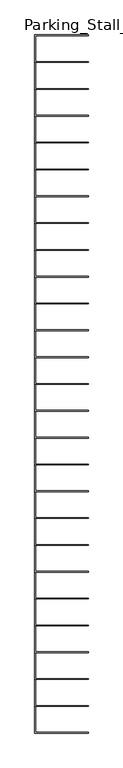
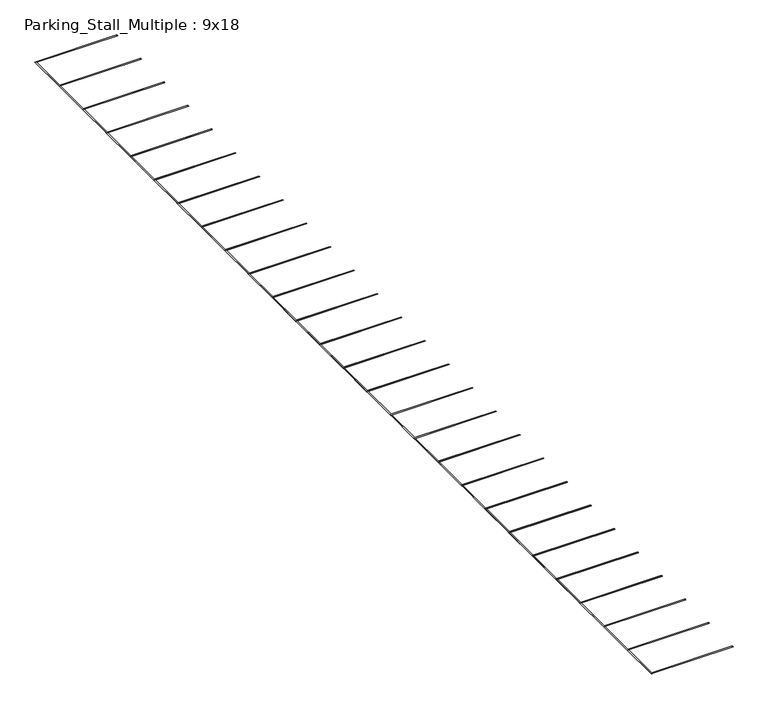
"""IFC4 building model written with IfcOpenShell, lengths in millimetres: proxy geometry, Parking_Stall_Multiple : 9x18."""

import ifcopenshell
import ifcopenshell.guid

model = None  # the IFC model being written
_history = None  # IfcOwnerHistory: only IFC2X3 demands one
_inside = {}  # id of a spatial element -> (the spatial element, [elements in it])
_under = {}  # id of a project, library or spatial element -> (it, [spatial elements below it])
_declared = {}  # id of a project -> (the project, [libraries it declares])
_typed = {}  # id of a type object -> (the type object, [elements of that type])
_made_of = {}  # id of a material, layer set ... -> (it, [elements and type objects made of it])


def new_model(schema):
    """Start an empty IFC model of exactly this schema.

    Asked for "IFC4X3", IfcOpenShell would pick the latest addendum, in which some entities
    have other attributes; the version numbers below select the first issue.
    IFC2X3 requires an IfcOwnerHistory on every rooted entity: one is made here for all.
    """
    global model, _history
    if schema == "IFC4X3":
        model = ifcopenshell.file(schema_version=(4, 3, 0, 0))
    else:
        model = ifcopenshell.file(schema=schema)
    _inside.clear()
    _under.clear()
    _declared.clear()
    _typed.clear()
    _made_of.clear()
    _history = None
    if model.schema == "IFC2X3":
        org = make("IfcOrganization", Name="unknown")
        user = make(
            "IfcPersonAndOrganization",
            ThePerson=make("IfcPerson", FamilyName="unknown"),
            TheOrganization=org,
        )
        app = make(
            "IfcApplication",
            ApplicationDeveloper=org,
            Version="unknown",
            ApplicationFullName="unknown",
            ApplicationIdentifier="unknown",
        )
        _history = make(
            "IfcOwnerHistory",
            OwningUser=user,
            OwningApplication=app,
            ChangeAction="ADDED",
            CreationDate=0,
        )
    return model


def make(cls, **values):
    """One entity of the class cls with the attributes given. An attribute that is None is left unset."""
    return model.create_entity(
        cls, **{name: value for name, value in values.items() if value is not None}
    )


def rooted(cls, **values):
    """An entity with a GlobalId (a new one), such as an element, a storey or a relation."""
    return make(cls, GlobalId=ifcopenshell.guid.new(), OwnerHistory=_history, **values)


def si_unit(unit_type, name, prefix=None):
    """IfcSIUnit, for example si_unit("LENGTHUNIT", "METRE", prefix="MILLI")."""
    return make("IfcSIUnit", UnitType=unit_type, Prefix=prefix, Name=name)


def assignment(units):
    """IfcUnitAssignment: the units of a project."""
    return None if units is None else make("IfcUnitAssignment", Units=units)


def point(xyz):
    """IfcCartesianPoint."""
    return None if xyz is None else make("IfcCartesianPoint", Coordinates=xyz)


def direction(xyz):
    """IfcDirection."""
    return None if xyz is None else make("IfcDirection", DirectionRatios=xyz)


def frame(location, z_axis=None, x_axis=None):
    """IfcAxis2Placement3D, a coordinate frame: its origin and axes. An axis left out is left unset."""
    return make(
        "IfcAxis2Placement3D",
        Location=point(location),
        Axis=direction(z_axis),
        RefDirection=direction(x_axis),
    )


def origin():
    """The frame at (0, 0, 0) with its axes left unset."""
    return frame((0.0, 0.0, 0.0))


def origin_with_axes():
    """The frame at (0, 0, 0) with the z axis (0, 0, 1) and the x axis (1, 0, 0) written out."""
    return frame((0.0, 0.0, 0.0), z_axis=(0.0, 0.0, 1.0), x_axis=(1.0, 0.0, 0.0))


def place(relative_to, where):
    """IfcLocalPlacement: puts the frame where relative to a parent placement (None: the world)."""
    return make(
        "IfcLocalPlacement", PlacementRelTo=relative_to, RelativePlacement=where
    )


def context(
    kind, dimensions, precision=None, world=None, true_north=None, identifier=None
):
    """IfcGeometricRepresentationContext, for example the 3D "Model" context."""
    return make(
        "IfcGeometricRepresentationContext",
        ContextIdentifier=identifier,
        ContextType=kind,
        CoordinateSpaceDimension=dimensions,
        Precision=precision,
        WorldCoordinateSystem=world,
        TrueNorth=true_north,
    )


def project(units=None, contexts=None):
    """IfcProject with its units and contexts."""
    return rooted(
        "IfcProject",
        Name="project",
        RepresentationContexts=contexts,
        UnitsInContext=assignment(units),
    )


def spatial(cls, under=None, at=None, **own):
    """A site, building, storey or space (cls), placed at a placement, below another one or the project."""
    s = rooted(cls, ObjectPlacement=at, **own)
    if under is not None:
        _under.setdefault(under.id(), (under, []))[1].append(s)
    return s


def polyline(points):
    """IfcPolyline through the points."""
    return make("IfcPolyline", Points=[point(p) for p in points])


def outline(outer, holes=None, kind="AREA"):
    """IfcArbitraryClosedProfileDef: a profile drawn as a closed curve; with holes, ...WithVoids."""
    if holes is None:
        return make("IfcArbitraryClosedProfileDef", ProfileType=kind, OuterCurve=outer)
    return make(
        "IfcArbitraryProfileDefWithVoids",
        ProfileType=kind,
        OuterCurve=outer,
        InnerCurves=holes,
    )


def extrude(swept, where, along, depth):
    """IfcExtrudedAreaSolid: the profile swept, set in the frame where, extruded along a direction by depth."""
    return make(
        "IfcExtrudedAreaSolid",
        SweptArea=swept,
        Position=where,
        ExtrudedDirection=direction(along),
        Depth=depth,
    )


def shape(context_of_items, identifier, shape_type, items):
    """IfcShapeRepresentation: the items that make up one representation, for example the "Body"."""
    return make(
        "IfcShapeRepresentation",
        ContextOfItems=context_of_items,
        RepresentationIdentifier=identifier,
        RepresentationType=shape_type,
        Items=items,
    )


def source(mapping_origin, context_of_items, identifier, shape_type, items):
    """IfcRepresentationMap: a shape defined once, which mapped items show again and again."""
    return make(
        "IfcRepresentationMap",
        MappingOrigin=mapping_origin,
        MappedRepresentation=shape(context_of_items, identifier, shape_type, items),
    )


def transform(
    local_origin,
    x_axis=None,
    y_axis=None,
    z_axis=None,
    scale=None,
    scale2=None,
    scale3=None,
    uniform=True,
):
    """IfcCartesianTransformationOperator3D, or its non-uniform kind. x_axis, y_axis, z_axis: its Axis1, 2, 3."""
    if uniform:
        return make(
            "IfcCartesianTransformationOperator3D",
            Axis1=direction(x_axis),
            Axis2=direction(y_axis),
            LocalOrigin=point(local_origin),
            Scale=scale,
            Axis3=direction(z_axis),
        )
    return make(
        "IfcCartesianTransformationOperator3DnonUniform",
        Axis1=direction(x_axis),
        Axis2=direction(y_axis),
        LocalOrigin=point(local_origin),
        Scale=scale,
        Axis3=direction(z_axis),
        Scale2=scale2,
        Scale3=scale3,
    )


def mapped(mapping_source, mapping_target):
    """IfcMappedItem: shows the shape of a source again, moved by a transform."""
    return make(
        "IfcMappedItem", MappingSource=mapping_source, MappingTarget=mapping_target
    )


def made_of(thing, what):
    """Note that an element or type object is made of a material, layer set ...; save() writes the relation."""
    if what is not None:
        _made_of.setdefault(what.id(), (what, []))[1].append(thing)
    return thing


def element(
    cls,
    number,
    at=None,
    inside=None,
    cuts=None,
    type_object=None,
    material=None,
    context=None,
    identifier="Body",
    shape_type=None,
    held_by="IfcProductDefinitionShape",
    body=None,
    shapes=None,
    **own,
):
    """One element of the class cls, such as IfcWall. Its Tag is "e" and its number.

    at: its placement. inside: the storey or other place that contains it. cuts: it is an
    opening in that element (IfcRelVoidsElement). A single representation is given by context,
    identifier, shape_type and body (its items); several are given by shapes. held_by: the class
    of the entity that holds the representations. save() writes the other relations.
    """
    e = rooted(cls, Tag="e%d" % number, ObjectPlacement=at, **own)
    if body is not None:
        shapes = [shape(context, identifier, shape_type, body)]
    if shapes is not None:
        e.Representation = make(held_by, Representations=shapes)
    if inside is not None:
        _inside.setdefault(inside.id(), (inside, []))[1].append(e)
    if cuts is not None:
        rooted(
            "IfcRelVoidsElement", RelatingBuildingElement=cuts, RelatedOpeningElement=e
        )
    if type_object is not None:
        _typed.setdefault(type_object.id(), (type_object, []))[1].append(e)
    return made_of(e, material)


def aggregate(whole, parts):
    """IfcRelAggregates: a whole, such as a stair, and the parts it consists of."""
    return rooted("IfcRelAggregates", RelatingObject=whole, RelatedObjects=parts)


def save(model, path):
    """Write the relations noted so far, then the file.

    IfcRelAggregates (storeys below a building ...), IfcRelContainedInSpatialStructure (elements
    in a storey), IfcRelDefinesByType, IfcRelAssociatesMaterial and IfcRelDeclares: one each for
    every whole, place, type object, material and project.
    """
    for whole, parts in _under.values():
        aggregate(whole, parts)
    for where, things in _inside.values():
        rooted(
            "IfcRelContainedInSpatialStructure",
            RelatedElements=things,
            RelatingStructure=where,
        )
    for kind, things in _typed.values():
        rooted("IfcRelDefinesByType", RelatedObjects=things, RelatingType=kind)
    for what, things in _made_of.values():
        rooted("IfcRelAssociatesMaterial", RelatedObjects=things, RelatingMaterial=what)
    for by, libraries in _declared.values():
        rooted("IfcRelDeclares", RelatingContext=by, RelatedDefinitions=libraries)
    model.write(path)


def parking_stall_multiple_9x18_b666618d(model_context):
    return source(origin(), model_context, "Body", "SweptSolid", [
        extrude(outline(polyline([(5486.4, 68580.0), (0.0, 68580.0), (0.0, 71399.4), (5486.4, 71399.4), (5486.4, 71323.2), (76.2, 71323.2), (76.2, 68656.2), (5486.4, 68656.2), (5486.4, 68580.0)])), origin_with_axes(), (0.0, 0.0, 1.0), 6.35),
        extrude(outline(polyline([(5486.4, 65836.8), (0.0, 65836.8), (0.0, 68656.2), (5486.4, 68656.2), (5486.4, 68580.0), (76.2, 68580.0), (76.2, 65913.0), (5486.4, 65913.0), (5486.4, 65836.8)])), origin_with_axes(), (0.0, 0.0, 1.0), 6.35),
        extrude(outline(polyline([(5486.4, 63093.6), (0.0, 63093.6), (0.0, 65913.0), (5486.4, 65913.0), (5486.4, 65836.8), (76.2, 65836.8), (76.2, 63169.8), (5486.4, 63169.8), (5486.4, 63093.6)])), origin_with_axes(), (0.0, 0.0, 1.0), 6.35),
        extrude(outline(polyline([(5486.4, 60350.4), (0.0, 60350.4), (0.0, 63169.8), (5486.4, 63169.8), (5486.4, 63093.6), (76.2, 63093.6), (76.2, 60426.6), (5486.4, 60426.6), (5486.4, 60350.4)])), origin_with_axes(), (0.0, 0.0, 1.0), 6.35),
        extrude(outline(polyline([(5486.4, 57607.2), (0.0, 57607.2), (0.0, 60426.6), (5486.4, 60426.6), (5486.4, 60350.4), (76.2, 60350.4), (76.2, 57683.4), (5486.4, 57683.4), (5486.4, 57607.2)])), origin_with_axes(), (0.0, 0.0, 1.0), 6.35),
        extrude(outline(polyline([(5486.4, 54864.0), (0.0, 54864.0), (0.0, 57683.4), (5486.4, 57683.4), (5486.4, 57607.2), (76.2, 57607.2), (76.2, 54940.2), (5486.4, 54940.2), (5486.4, 54864.0)])), origin_with_axes(), (0.0, 0.0, 1.0), 6.35),
        extrude(outline(polyline([(5486.4, 52120.8), (0.0, 52120.8), (0.0, 54940.2), (5486.4, 54940.2), (5486.4, 54864.0), (76.2, 54864.0), (76.2, 52197.0), (5486.4, 52197.0), (5486.4, 52120.8)])), origin_with_axes(), (0.0, 0.0, 1.0), 6.35),
        extrude(outline(polyline([(5486.4, 49377.6), (0.0, 49377.6), (0.0, 52197.0), (5486.4, 52197.0), (5486.4, 52120.8), (76.2, 52120.8), (76.2, 49453.8), (5486.4, 49453.8), (5486.4, 49377.6)])), origin_with_axes(), (0.0, 0.0, 1.0), 6.35),
        extrude(outline(polyline([(5486.4, 46634.4), (0.0, 46634.4), (0.0, 49453.8), (5486.4, 49453.8), (5486.4, 49377.6), (76.2, 49377.6), (76.2, 46710.6), (5486.4, 46710.6), (5486.4, 46634.4)])), origin_with_axes(), (0.0, 0.0, 1.0), 6.35),
        extrude(outline(polyline([(5486.4, 43891.2), (0.0, 43891.2), (0.0, 46710.6), (5486.4, 46710.6), (5486.4, 46634.4), (76.2, 46634.4), (76.2, 43967.4), (5486.4, 43967.4), (5486.4, 43891.2)])), origin_with_axes(), (0.0, 0.0, 1.0), 6.35),
        extrude(outline(polyline([(5486.4, 41148.0), (0.0, 41148.0), (0.0, 43967.4), (5486.4, 43967.4), (5486.4, 43891.2), (76.2, 43891.2), (76.2, 41224.2), (5486.4, 41224.2), (5486.4, 41148.0)])), origin_with_axes(), (0.0, 0.0, 1.0), 6.35),
        extrude(outline(polyline([(5486.4, 38404.8), (0.0, 38404.8), (0.0, 41224.2), (5486.4, 41224.2), (5486.4, 41148.0), (76.2, 41148.0), (76.2, 38481.0), (5486.4, 38481.0), (5486.4, 38404.8)])), origin_with_axes(), (0.0, 0.0, 1.0), 6.35),
        extrude(outline(polyline([(5486.4, 35661.6), (0.0, 35661.6), (0.0, 38481.0), (5486.4, 38481.0), (5486.4, 38404.8), (76.2, 38404.8), (76.2, 35737.8), (5486.4, 35737.8), (5486.4, 35661.6)])), origin_with_axes(), (0.0, 0.0, 1.0), 6.35),
        extrude(outline(polyline([(5486.4, 32918.4), (0.0, 32918.4), (0.0, 35737.8), (5486.4, 35737.8), (5486.4, 35661.6), (76.2, 35661.6), (76.2, 32994.6), (5486.4, 32994.6), (5486.4, 32918.4)])), origin_with_axes(), (0.0, 0.0, 1.0), 6.35),
        extrude(outline(polyline([(5486.4, 30175.2), (0.0, 30175.2), (0.0, 32994.6), (5486.4, 32994.6), (5486.4, 32918.4), (76.2, 32918.4), (76.2, 30251.4), (5486.4, 30251.4), (5486.4, 30175.2)])), origin_with_axes(), (0.0, 0.0, 1.0), 6.35),
        extrude(outline(polyline([(5486.4, 27432.0), (0.0, 27432.0), (0.0, 30251.4), (5486.4, 30251.4), (5486.4, 30175.2), (76.2, 30175.2), (76.2, 27508.2), (5486.4, 27508.2), (5486.4, 27432.0)])), origin_with_axes(), (0.0, 0.0, 1.0), 6.35),
        extrude(outline(polyline([(5486.4, 24688.8), (0.0, 24688.8), (0.0, 27508.2), (5486.4, 27508.2), (5486.4, 27432.0), (76.2, 27432.0), (76.2, 24765.0), (5486.4, 24765.0), (5486.4, 24688.8)])), origin_with_axes(), (0.0, 0.0, 1.0), 6.35),
        extrude(outline(polyline([(5486.4, 21945.6), (0.0, 21945.6), (0.0, 24765.0), (5486.4, 24765.0), (5486.4, 24688.8), (76.2, 24688.8), (76.2, 22021.8), (5486.4, 22021.8), (5486.4, 21945.6)])), origin_with_axes(), (0.0, 0.0, 1.0), 6.35),
        extrude(outline(polyline([(5486.4, 19202.4), (0.0, 19202.4), (0.0, 22021.8), (5486.4, 22021.8), (5486.4, 21945.6), (76.2, 21945.6), (76.2, 19278.6), (5486.4, 19278.6), (5486.4, 19202.4)])), origin_with_axes(), (0.0, 0.0, 1.0), 6.35),
        extrude(outline(polyline([(5486.4, 16459.2), (0.0, 16459.2), (0.0, 19278.6), (5486.4, 19278.6), (5486.4, 19202.4), (76.2, 19202.4), (76.2, 16535.4), (5486.4, 16535.4), (5486.4, 16459.2)])), origin_with_axes(), (0.0, 0.0, 1.0), 6.35),
        extrude(outline(polyline([(5486.4, 13716.0), (0.0, 13716.0), (0.0, 16535.4), (5486.4, 16535.4), (5486.4, 16459.2), (76.2, 16459.2), (76.2, 13792.2), (5486.4, 13792.2), (5486.4, 13716.0)])), origin_with_axes(), (0.0, 0.0, 1.0), 6.35),
        extrude(outline(polyline([(5486.4, 10972.8), (0.0, 10972.8), (0.0, 13792.2), (5486.4, 13792.2), (5486.4, 13716.0), (76.2, 13716.0), (76.2, 11049.0), (5486.4, 11049.0), (5486.4, 10972.8)])), origin_with_axes(), (0.0, 0.0, 1.0), 6.35),
        extrude(outline(polyline([(5486.4, 8229.6), (0.0, 8229.6), (0.0, 11049.0), (5486.4, 11049.0), (5486.4, 10972.8), (76.2, 10972.8), (76.2, 8305.8), (5486.4, 8305.8), (5486.4, 8229.6)])), origin_with_axes(), (0.0, 0.0, 1.0), 6.35),
        extrude(outline(polyline([(5486.4, 5486.4), (0.0, 5486.4), (0.0, 8305.8), (5486.4, 8305.8), (5486.4, 8229.6), (76.2, 8229.6), (76.2, 5562.6), (5486.4, 5562.6), (5486.4, 5486.4)])), origin_with_axes(), (0.0, 0.0, 1.0), 6.35),
        extrude(outline(polyline([(5486.4, 2743.2), (0.0, 2743.2), (0.0, 5562.6), (5486.4, 5562.6), (5486.4, 5486.4), (76.2, 5486.4), (76.2, 2819.4), (5486.4, 2819.4), (5486.4, 2743.2)])), origin_with_axes(), (0.0, 0.0, 1.0), 6.35),
        extrude(outline(polyline([(5486.4, 0.0), (0.0, 0.0), (0.0, 2819.4), (5486.4, 2819.4), (5486.4, 2743.2), (76.2, 2743.2), (76.2, 76.2), (5486.4, 76.2), (5486.4, 0.0)])), origin_with_axes(), (0.0, 0.0, 1.0), 6.35),
    ])


if __name__ == "__main__":
    model = new_model("IFC4")
    model_context = context("Model", 3, world=origin())
    ifc_project = project(units=[si_unit("LENGTHUNIT", "METRE", prefix="MILLI")], contexts=[model_context])
    site = spatial("IfcSite", under=ifc_project)
    building = spatial("IfcBuilding", under=site)
    placement = place(None, origin())
    parking_stall_multiple_9x18_shape = parking_stall_multiple_9x18_b666618d(model_context)
    element("IfcBuildingElementProxy", 1, Name="Parking_Stall_Multiple : 9x18", ObjectType="Parking_Stall_Multiple : 9x18", at=placement, inside=building, context=model_context, shape_type="MappedRepresentation", body=[
        mapped(parking_stall_multiple_9x18_shape, transform((0.0, 0.0, 0.0), x_axis=(1.0, 0.0, 0.0), y_axis=(0.0, 1.0, 0.0), z_axis=(0.0, 0.0, 1.0))),
    ])
    save(model, "model.ifc")

# Revit data of these elements
# Type "Parking_Stall_Multiple : 9x18"
#   Parking_Width_M = 9' - 0"
#   Parking_Run_Length [instance default] = 65' - 0"
#   Parking_Line_Width = 0' - 3"
#   Parking_Length_M = 18' - 0"
#   Single_Parking_Visibility [instance default] = no
#   Parking_ADA_Symbol = no
#   ParkingUnitsArray [instance default] = 7
#   ParkingUnits [instance default] = 7
#   Multiple_Parking_Visibility [instance default] = yes
#   Parking_Line_Material = none
# Element 1 (IfcBuildingElementProxy, "Parking_Stall_Multiple : 9x18")
#   Parking_Run_Length = 238' - 3.19592"
#   ParkingUnitsArray = 26
#   ParkingUnits = 26
